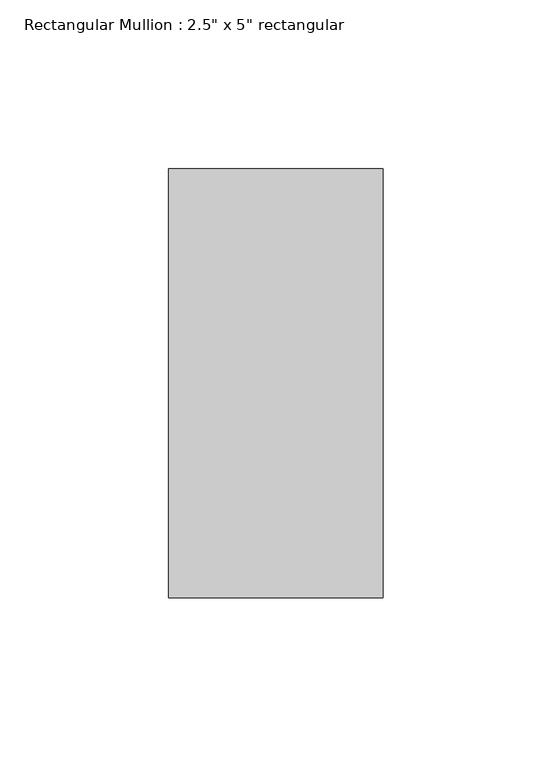
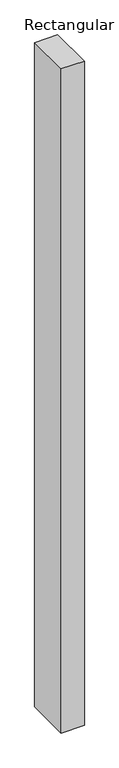
"""IFC4 building model written with IfcOpenShell, lengths in millimetres: member geometry."""

import ifcopenshell
import ifcopenshell.guid

model = None  # the IFC model being written
_history = None  # IfcOwnerHistory: only IFC2X3 demands one
_inside = {}  # id of a spatial element -> (the spatial element, [elements in it])
_under = {}  # id of a project, library or spatial element -> (it, [spatial elements below it])
_declared = {}  # id of a project -> (the project, [libraries it declares])
_typed = {}  # id of a type object -> (the type object, [elements of that type])
_made_of = {}  # id of a material, layer set ... -> (it, [elements and type objects made of it])


def new_model(schema):
    """Start an empty IFC model of exactly this schema.

    Asked for "IFC4X3", IfcOpenShell would pick the latest addendum, in which some entities
    have other attributes; the version numbers below select the first issue.
    IFC2X3 requires an IfcOwnerHistory on every rooted entity: one is made here for all.
    """
    global model, _history
    if schema == "IFC4X3":
        model = ifcopenshell.file(schema_version=(4, 3, 0, 0))
    else:
        model = ifcopenshell.file(schema=schema)
    _inside.clear()
    _under.clear()
    _declared.clear()
    _typed.clear()
    _made_of.clear()
    _history = None
    if model.schema == "IFC2X3":
        org = make("IfcOrganization", Name="unknown")
        user = make(
            "IfcPersonAndOrganization",
            ThePerson=make("IfcPerson", FamilyName="unknown"),
            TheOrganization=org,
        )
        app = make(
            "IfcApplication",
            ApplicationDeveloper=org,
            Version="unknown",
            ApplicationFullName="unknown",
            ApplicationIdentifier="unknown",
        )
        _history = make(
            "IfcOwnerHistory",
            OwningUser=user,
            OwningApplication=app,
            ChangeAction="ADDED",
            CreationDate=0,
        )
    return model


def make(cls, **values):
    """One entity of the class cls with the attributes given. An attribute that is None is left unset."""
    return model.create_entity(
        cls, **{name: value for name, value in values.items() if value is not None}
    )


def rooted(cls, **values):
    """An entity with a GlobalId (a new one), such as an element, a storey or a relation."""
    return make(cls, GlobalId=ifcopenshell.guid.new(), OwnerHistory=_history, **values)


def si_unit(unit_type, name, prefix=None):
    """IfcSIUnit, for example si_unit("LENGTHUNIT", "METRE", prefix="MILLI")."""
    return make("IfcSIUnit", UnitType=unit_type, Prefix=prefix, Name=name)


def assignment(units):
    """IfcUnitAssignment: the units of a project."""
    return None if units is None else make("IfcUnitAssignment", Units=units)


def point(xyz):
    """IfcCartesianPoint."""
    return None if xyz is None else make("IfcCartesianPoint", Coordinates=xyz)


def direction(xyz):
    """IfcDirection."""
    return None if xyz is None else make("IfcDirection", DirectionRatios=xyz)


def frame(location, z_axis=None, x_axis=None):
    """IfcAxis2Placement3D, a coordinate frame: its origin and axes. An axis left out is left unset."""
    return make(
        "IfcAxis2Placement3D",
        Location=point(location),
        Axis=direction(z_axis),
        RefDirection=direction(x_axis),
    )


def origin():
    """The frame at (0, 0, 0) with its axes left unset."""
    return frame((0.0, 0.0, 0.0))


def place(relative_to, where):
    """IfcLocalPlacement: puts the frame where relative to a parent placement (None: the world)."""
    return make(
        "IfcLocalPlacement", PlacementRelTo=relative_to, RelativePlacement=where
    )


def context(
    kind, dimensions, precision=None, world=None, true_north=None, identifier=None
):
    """IfcGeometricRepresentationContext, for example the 3D "Model" context."""
    return make(
        "IfcGeometricRepresentationContext",
        ContextIdentifier=identifier,
        ContextType=kind,
        CoordinateSpaceDimension=dimensions,
        Precision=precision,
        WorldCoordinateSystem=world,
        TrueNorth=true_north,
    )


def project(units=None, contexts=None):
    """IfcProject with its units and contexts."""
    return rooted(
        "IfcProject",
        Name="project",
        RepresentationContexts=contexts,
        UnitsInContext=assignment(units),
    )


def spatial(cls, under=None, at=None, **own):
    """A site, building, storey or space (cls), placed at a placement, below another one or the project."""
    s = rooted(cls, ObjectPlacement=at, **own)
    if under is not None:
        _under.setdefault(under.id(), (under, []))[1].append(s)
    return s


def polyline(points):
    """IfcPolyline through the points."""
    return make("IfcPolyline", Points=[point(p) for p in points])


def outline(outer, holes=None, kind="AREA"):
    """IfcArbitraryClosedProfileDef: a profile drawn as a closed curve; with holes, ...WithVoids."""
    if holes is None:
        return make("IfcArbitraryClosedProfileDef", ProfileType=kind, OuterCurve=outer)
    return make(
        "IfcArbitraryProfileDefWithVoids",
        ProfileType=kind,
        OuterCurve=outer,
        InnerCurves=holes,
    )


def extrude(swept, where, along, depth):
    """IfcExtrudedAreaSolid: the profile swept, set in the frame where, extruded along a direction by depth."""
    return make(
        "IfcExtrudedAreaSolid",
        SweptArea=swept,
        Position=where,
        ExtrudedDirection=direction(along),
        Depth=depth,
    )


def shape(context_of_items, identifier, shape_type, items):
    """IfcShapeRepresentation: the items that make up one representation, for example the "Body"."""
    return make(
        "IfcShapeRepresentation",
        ContextOfItems=context_of_items,
        RepresentationIdentifier=identifier,
        RepresentationType=shape_type,
        Items=items,
    )


def source(mapping_origin, context_of_items, identifier, shape_type, items):
    """IfcRepresentationMap: a shape defined once, which mapped items show again and again."""
    return make(
        "IfcRepresentationMap",
        MappingOrigin=mapping_origin,
        MappedRepresentation=shape(context_of_items, identifier, shape_type, items),
    )


def transform(
    local_origin,
    x_axis=None,
    y_axis=None,
    z_axis=None,
    scale=None,
    scale2=None,
    scale3=None,
    uniform=True,
):
    """IfcCartesianTransformationOperator3D, or its non-uniform kind. x_axis, y_axis, z_axis: its Axis1, 2, 3."""
    if uniform:
        return make(
            "IfcCartesianTransformationOperator3D",
            Axis1=direction(x_axis),
            Axis2=direction(y_axis),
            LocalOrigin=point(local_origin),
            Scale=scale,
            Axis3=direction(z_axis),
        )
    return make(
        "IfcCartesianTransformationOperator3DnonUniform",
        Axis1=direction(x_axis),
        Axis2=direction(y_axis),
        LocalOrigin=point(local_origin),
        Scale=scale,
        Axis3=direction(z_axis),
        Scale2=scale2,
        Scale3=scale3,
    )


def mapped(mapping_source, mapping_target):
    """IfcMappedItem: shows the shape of a source again, moved by a transform."""
    return make(
        "IfcMappedItem", MappingSource=mapping_source, MappingTarget=mapping_target
    )


def made_of(thing, what):
    """Note that an element or type object is made of a material, layer set ...; save() writes the relation."""
    if what is not None:
        _made_of.setdefault(what.id(), (what, []))[1].append(thing)
    return thing


def element(
    cls,
    number,
    at=None,
    inside=None,
    cuts=None,
    type_object=None,
    material=None,
    context=None,
    identifier="Body",
    shape_type=None,
    held_by="IfcProductDefinitionShape",
    body=None,
    shapes=None,
    **own,
):
    """One element of the class cls, such as IfcWall. Its Tag is "e" and its number.

    at: its placement. inside: the storey or other place that contains it. cuts: it is an
    opening in that element (IfcRelVoidsElement). A single representation is given by context,
    identifier, shape_type and body (its items); several are given by shapes. held_by: the class
    of the entity that holds the representations. save() writes the other relations.
    """
    e = rooted(cls, Tag="e%d" % number, ObjectPlacement=at, **own)
    if body is not None:
        shapes = [shape(context, identifier, shape_type, body)]
    if shapes is not None:
        e.Representation = make(held_by, Representations=shapes)
    if inside is not None:
        _inside.setdefault(inside.id(), (inside, []))[1].append(e)
    if cuts is not None:
        rooted(
            "IfcRelVoidsElement", RelatingBuildingElement=cuts, RelatedOpeningElement=e
        )
    if type_object is not None:
        _typed.setdefault(type_object.id(), (type_object, []))[1].append(e)
    return made_of(e, material)


def aggregate(whole, parts):
    """IfcRelAggregates: a whole, such as a stair, and the parts it consists of."""
    return rooted("IfcRelAggregates", RelatingObject=whole, RelatedObjects=parts)


def save(model, path):
    """Write the relations noted so far, then the file.

    IfcRelAggregates (storeys below a building ...), IfcRelContainedInSpatialStructure (elements
    in a storey), IfcRelDefinesByType, IfcRelAssociatesMaterial and IfcRelDeclares: one each for
    every whole, place, type object, material and project.
    """
    for whole, parts in _under.values():
        aggregate(whole, parts)
    for where, things in _inside.values():
        rooted(
            "IfcRelContainedInSpatialStructure",
            RelatedElements=things,
            RelatingStructure=where,
        )
    for kind, things in _typed.values():
        rooted("IfcRelDefinesByType", RelatedObjects=things, RelatingType=kind)
    for what, things in _made_of.values():
        rooted("IfcRelAssociatesMaterial", RelatedObjects=things, RelatingMaterial=what)
    for by, libraries in _declared.values():
        rooted("IfcRelDeclares", RelatingContext=by, RelatedDefinitions=libraries)
    model.write(path)


def member_7a85b04f(model_context):
    return source(origin(), model_context, "Body", "SweptSolid", [
        extrude(outline(polyline([(31.75, 63.5), (31.75, -63.5), (-31.75, -63.5), (-31.75, 63.5), (31.75, 63.5)])), frame((0.0, 0.0, -1936.75), z_axis=(0.0, 0.0, 1.0), x_axis=(1.0, 0.0, 0.0)), (0.0, 0.0, 1.0), 1936.75),
    ])


if __name__ == "__main__":
    model = new_model("IFC4")
    model_context = context("Model", 3, world=origin())
    ifc_project = project(units=[si_unit("LENGTHUNIT", "METRE", prefix="MILLI")], contexts=[model_context])
    site = spatial("IfcSite", under=ifc_project)
    building = spatial("IfcBuilding", under=site)
    placement = place(None, origin())
    member_shape = member_7a85b04f(model_context)
    element("IfcMember", 1, ObjectType="Rectangular Mullion : 2.5\" x 5\" rectangular", at=placement, inside=building, context=model_context, shape_type="MappedRepresentation", body=[
        mapped(member_shape, transform((0.0, 0.0, 0.0), x_axis=(1.0, 0.0, 0.0), y_axis=(0.0, 1.0, 0.0), z_axis=(0.0, 0.0, 1.0))),
    ])
    save(model, "model.ifc")

# Revit data of these elements
# Type "Rectangular Mullion : 2.5\" x 5\" rectangular"
#   built-in parameter 1007304 = 0.416667 (stored number, unit not read)
#   built-in parameter 1007301 = 0.104167 (stored number, unit not read)
#   built-in parameter 1007300 = 0.104167 (stored number, unit not read)
# Element 1 (IfcMember, "Rectangular Mullion : 2.5\" x 5\" rectangular")
#   Materials on its faces: "Metal - Aluminum"
# Materials
#   "Metal - Aluminum": class "Metal", colour RGB 140 140 140, transparency 0
